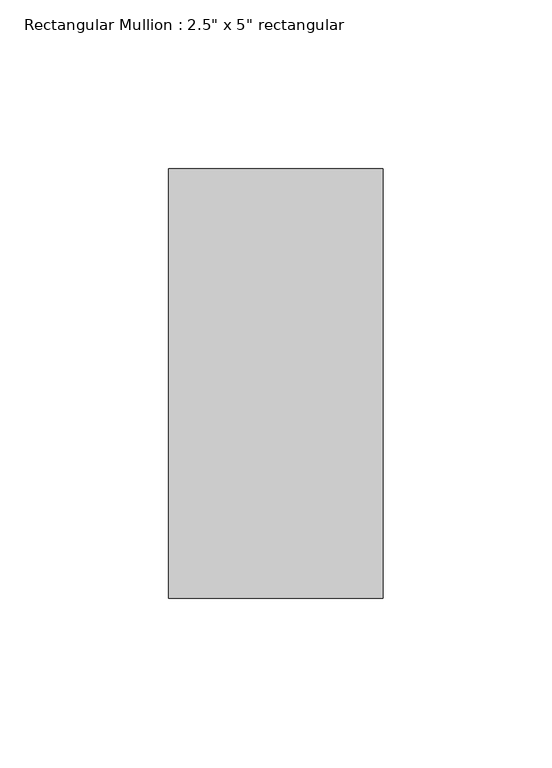
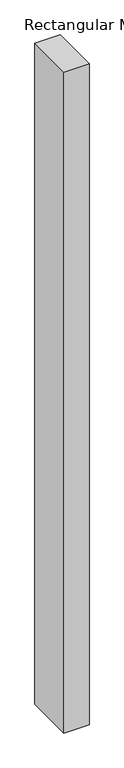
"""IFC4 building model written with IfcOpenShell, lengths in millimetres: member geometry."""

import ifcopenshell
import ifcopenshell.guid

model = None  # the IFC model being written
_history = None  # IfcOwnerHistory: only IFC2X3 demands one
_inside = {}  # id of a spatial element -> (the spatial element, [elements in it])
_under = {}  # id of a project, library or spatial element -> (it, [spatial elements below it])
_declared = {}  # id of a project -> (the project, [libraries it declares])
_typed = {}  # id of a type object -> (the type object, [elements of that type])
_made_of = {}  # id of a material, layer set ... -> (it, [elements and type objects made of it])


def new_model(schema):
    """Start an empty IFC model of exactly this schema.

    Asked for "IFC4X3", IfcOpenShell would pick the latest addendum, in which some entities
    have other attributes; the version numbers below select the first issue.
    IFC2X3 requires an IfcOwnerHistory on every rooted entity: one is made here for all.
    """
    global model, _history
    if schema == "IFC4X3":
        model = ifcopenshell.file(schema_version=(4, 3, 0, 0))
    else:
        model = ifcopenshell.file(schema=schema)
    _inside.clear()
    _under.clear()
    _declared.clear()
    _typed.clear()
    _made_of.clear()
    _history = None
    if model.schema == "IFC2X3":
        org = make("IfcOrganization", Name="unknown")
        user = make(
            "IfcPersonAndOrganization",
            ThePerson=make("IfcPerson", FamilyName="unknown"),
            TheOrganization=org,
        )
        app = make(
            "IfcApplication",
            ApplicationDeveloper=org,
            Version="unknown",
            ApplicationFullName="unknown",
            ApplicationIdentifier="unknown",
        )
        _history = make(
            "IfcOwnerHistory",
            OwningUser=user,
            OwningApplication=app,
            ChangeAction="ADDED",
            CreationDate=0,
        )
    return model


def make(cls, **values):
    """One entity of the class cls with the attributes given. An attribute that is None is left unset."""
    return model.create_entity(
        cls, **{name: value for name, value in values.items() if value is not None}
    )


def rooted(cls, **values):
    """An entity with a GlobalId (a new one), such as an element, a storey or a relation."""
    return make(cls, GlobalId=ifcopenshell.guid.new(), OwnerHistory=_history, **values)


def si_unit(unit_type, name, prefix=None):
    """IfcSIUnit, for example si_unit("LENGTHUNIT", "METRE", prefix="MILLI")."""
    return make("IfcSIUnit", UnitType=unit_type, Prefix=prefix, Name=name)


def assignment(units):
    """IfcUnitAssignment: the units of a project."""
    return None if units is None else make("IfcUnitAssignment", Units=units)


def point(xyz):
    """IfcCartesianPoint."""
    return None if xyz is None else make("IfcCartesianPoint", Coordinates=xyz)


def direction(xyz):
    """IfcDirection."""
    return None if xyz is None else make("IfcDirection", DirectionRatios=xyz)


def frame(location, z_axis=None, x_axis=None):
    """IfcAxis2Placement3D, a coordinate frame: its origin and axes. An axis left out is left unset."""
    return make(
        "IfcAxis2Placement3D",
        Location=point(location),
        Axis=direction(z_axis),
        RefDirection=direction(x_axis),
    )


def origin():
    """The frame at (0, 0, 0) with its axes left unset."""
    return frame((0.0, 0.0, 0.0))


def place(relative_to, where):
    """IfcLocalPlacement: puts the frame where relative to a parent placement (None: the world)."""
    return make(
        "IfcLocalPlacement", PlacementRelTo=relative_to, RelativePlacement=where
    )


def context(
    kind, dimensions, precision=None, world=None, true_north=None, identifier=None
):
    """IfcGeometricRepresentationContext, for example the 3D "Model" context."""
    return make(
        "IfcGeometricRepresentationContext",
        ContextIdentifier=identifier,
        ContextType=kind,
        CoordinateSpaceDimension=dimensions,
        Precision=precision,
        WorldCoordinateSystem=world,
        TrueNorth=true_north,
    )


def project(units=None, contexts=None):
    """IfcProject with its units and contexts."""
    return rooted(
        "IfcProject",
        Name="project",
        RepresentationContexts=contexts,
        UnitsInContext=assignment(units),
    )


def spatial(cls, under=None, at=None, **own):
    """A site, building, storey or space (cls), placed at a placement, below another one or the project."""
    s = rooted(cls, ObjectPlacement=at, **own)
    if under is not None:
        _under.setdefault(under.id(), (under, []))[1].append(s)
    return s


def polyline(points):
    """IfcPolyline through the points."""
    return make("IfcPolyline", Points=[point(p) for p in points])


def outline(outer, holes=None, kind="AREA"):
    """IfcArbitraryClosedProfileDef: a profile drawn as a closed curve; with holes, ...WithVoids."""
    if holes is None:
        return make("IfcArbitraryClosedProfileDef", ProfileType=kind, OuterCurve=outer)
    return make(
        "IfcArbitraryProfileDefWithVoids",
        ProfileType=kind,
        OuterCurve=outer,
        InnerCurves=holes,
    )


def extrude(swept, where, along, depth):
    """IfcExtrudedAreaSolid: the profile swept, set in the frame where, extruded along a direction by depth."""
    return make(
        "IfcExtrudedAreaSolid",
        SweptArea=swept,
        Position=where,
        ExtrudedDirection=direction(along),
        Depth=depth,
    )


def shape(context_of_items, identifier, shape_type, items):
    """IfcShapeRepresentation: the items that make up one representation, for example the "Body"."""
    return make(
        "IfcShapeRepresentation",
        ContextOfItems=context_of_items,
        RepresentationIdentifier=identifier,
        RepresentationType=shape_type,
        Items=items,
    )


def source(mapping_origin, context_of_items, identifier, shape_type, items):
    """IfcRepresentationMap: a shape defined once, which mapped items show again and again."""
    return make(
        "IfcRepresentationMap",
        MappingOrigin=mapping_origin,
        MappedRepresentation=shape(context_of_items, identifier, shape_type, items),
    )


def transform(
    local_origin,
    x_axis=None,
    y_axis=None,
    z_axis=None,
    scale=None,
    scale2=None,
    scale3=None,
    uniform=True,
):
    """IfcCartesianTransformationOperator3D, or its non-uniform kind. x_axis, y_axis, z_axis: its Axis1, 2, 3."""
    if uniform:
        return make(
            "IfcCartesianTransformationOperator3D",
            Axis1=direction(x_axis),
            Axis2=direction(y_axis),
            LocalOrigin=point(local_origin),
            Scale=scale,
            Axis3=direction(z_axis),
        )
    return make(
        "IfcCartesianTransformationOperator3DnonUniform",
        Axis1=direction(x_axis),
        Axis2=direction(y_axis),
        LocalOrigin=point(local_origin),
        Scale=scale,
        Axis3=direction(z_axis),
        Scale2=scale2,
        Scale3=scale3,
    )


def mapped(mapping_source, mapping_target):
    """IfcMappedItem: shows the shape of a source again, moved by a transform."""
    return make(
        "IfcMappedItem", MappingSource=mapping_source, MappingTarget=mapping_target
    )


def made_of(thing, what):
    """Note that an element or type object is made of a material, layer set ...; save() writes the relation."""
    if what is not None:
        _made_of.setdefault(what.id(), (what, []))[1].append(thing)
    return thing


def element(
    cls,
    number,
    at=None,
    inside=None,
    cuts=None,
    type_object=None,
    material=None,
    context=None,
    identifier="Body",
    shape_type=None,
    held_by="IfcProductDefinitionShape",
    body=None,
    shapes=None,
    **own,
):
    """One element of the class cls, such as IfcWall. Its Tag is "e" and its number.

    at: its placement. inside: the storey or other place that contains it. cuts: it is an
    opening in that element (IfcRelVoidsElement). A single representation is given by context,
    identifier, shape_type and body (its items); several are given by shapes. held_by: the class
    of the entity that holds the representations. save() writes the other relations.
    """
    e = rooted(cls, Tag="e%d" % number, ObjectPlacement=at, **own)
    if body is not None:
        shapes = [shape(context, identifier, shape_type, body)]
    if shapes is not None:
        e.Representation = make(held_by, Representations=shapes)
    if inside is not None:
        _inside.setdefault(inside.id(), (inside, []))[1].append(e)
    if cuts is not None:
        rooted(
            "IfcRelVoidsElement", RelatingBuildingElement=cuts, RelatedOpeningElement=e
        )
    if type_object is not None:
        _typed.setdefault(type_object.id(), (type_object, []))[1].append(e)
    return made_of(e, material)


def aggregate(whole, parts):
    """IfcRelAggregates: a whole, such as a stair, and the parts it consists of."""
    return rooted("IfcRelAggregates", RelatingObject=whole, RelatedObjects=parts)


def save(model, path):
    """Write the relations noted so far, then the file.

    IfcRelAggregates (storeys below a building ...), IfcRelContainedInSpatialStructure (elements
    in a storey), IfcRelDefinesByType, IfcRelAssociatesMaterial and IfcRelDeclares: one each for
    every whole, place, type object, material and project.
    """
    for whole, parts in _under.values():
        aggregate(whole, parts)
    for where, things in _inside.values():
        rooted(
            "IfcRelContainedInSpatialStructure",
            RelatedElements=things,
            RelatingStructure=where,
        )
    for kind, things in _typed.values():
        rooted("IfcRelDefinesByType", RelatedObjects=things, RelatingType=kind)
    for what, things in _made_of.values():
        rooted("IfcRelAssociatesMaterial", RelatedObjects=things, RelatingMaterial=what)
    for by, libraries in _declared.values():
        rooted("IfcRelDeclares", RelatingContext=by, RelatedDefinitions=libraries)
    model.write(path)


def member_6d5c3e5e(model_context):
    return source(origin(), model_context, "Body", "SweptSolid", [
        extrude(outline(polyline([(0.0, 63.5), (0.0, -63.5), (-63.5, -63.5), (-63.5, 63.5), (0.0, 63.5)])), frame((0.0, 0.0, -1765.3), z_axis=(0.0, 0.0, 1.0), x_axis=(1.0, 0.0, 0.0)), (0.0, 0.0, 1.0), 1765.3),
    ])


if __name__ == "__main__":
    model = new_model("IFC4")
    model_context = context("Model", 3, world=origin())
    ifc_project = project(units=[si_unit("LENGTHUNIT", "METRE", prefix="MILLI")], contexts=[model_context])
    site = spatial("IfcSite", under=ifc_project)
    building = spatial("IfcBuilding", under=site)
    placement = place(None, origin())
    member_shape = member_6d5c3e5e(model_context)
    element("IfcMember", 1, ObjectType="Rectangular Mullion : 2.5\" x 5\" rectangular", at=placement, inside=building, context=model_context, shape_type="MappedRepresentation", body=[
        mapped(member_shape, transform((0.0, 0.0, 0.0), x_axis=(1.0, 0.0, 0.0), y_axis=(0.0, 1.0, 0.0), z_axis=(0.0, 0.0, 1.0))),
    ])
    save(model, "model.ifc")

# Revit data of these elements
# Type "Rectangular Mullion : 2.5\" x 5\" rectangular"
#   built-in parameter 1007304 = 0.416667 (stored number, unit not read)
#   built-in parameter 1007301 = 0.104167 (stored number, unit not read)
#   built-in parameter 1007300 = 0.104167 (stored number, unit not read)
# Element 1 (IfcMember, "Rectangular Mullion : 2.5\" x 5\" rectangular")
#   Materials on its faces: "Aluminum"
# Materials
#   "Aluminum": class "Metal", colour RGB 247 247 247, transparency 0, Description = "Aluminum 6061", Cost = 0
